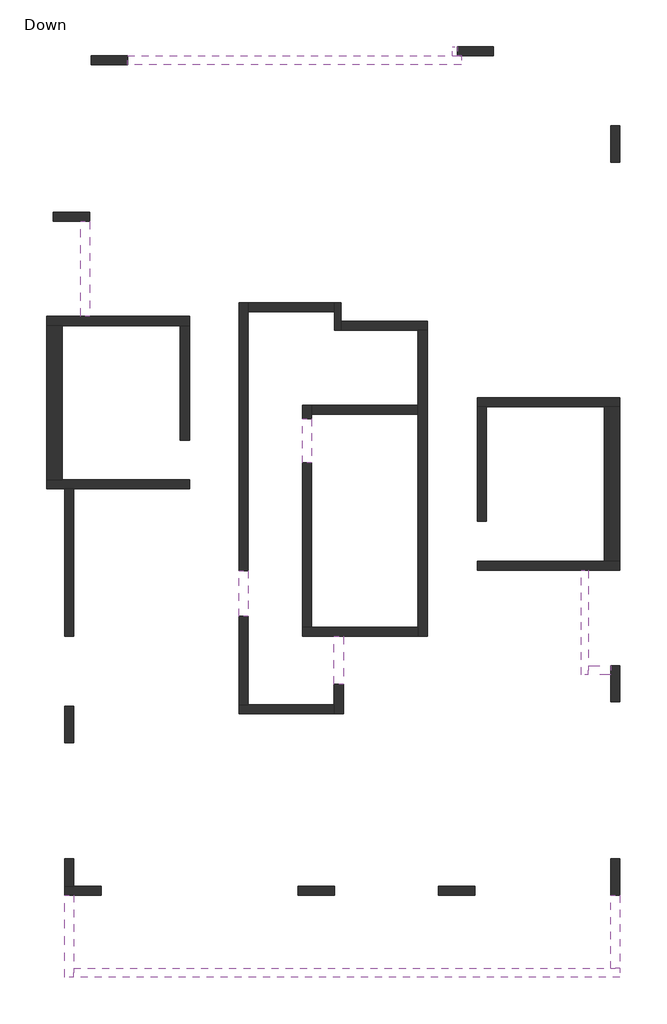
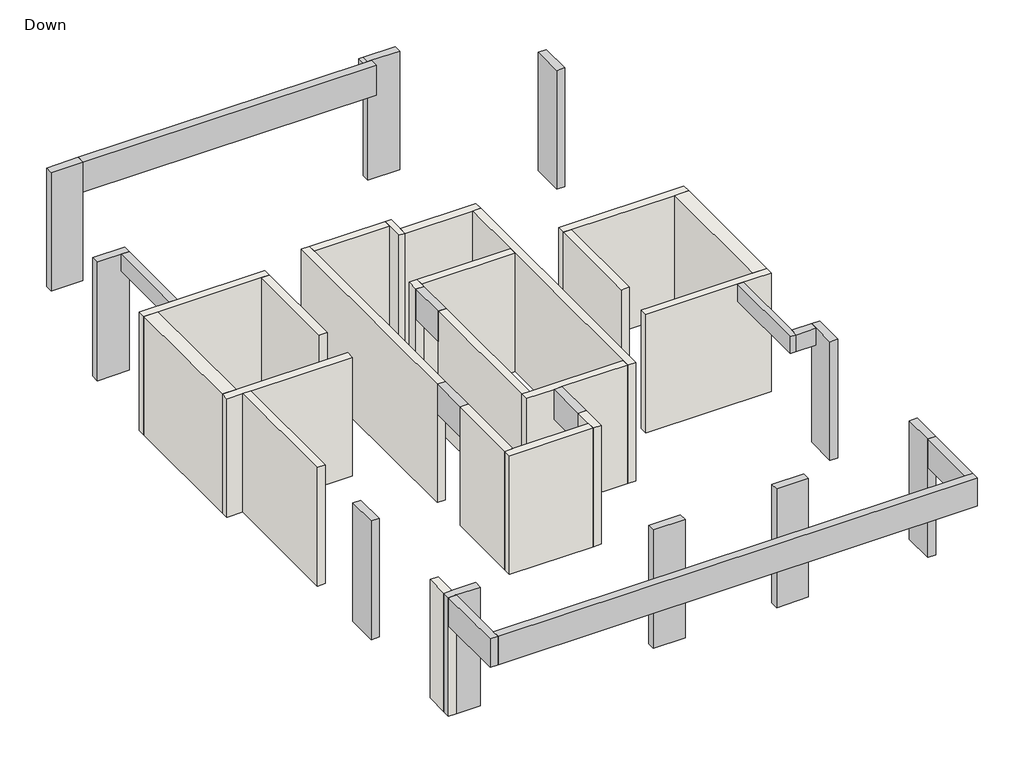
# One storey: 22 walls, 11 beams, 10 columns.
# Revit data of these elements (continued)
# Element 28 (IfcWall, "20") (continued)
#   SOFiSTiK_AMG_Adjusted = yes
#   Phase Created = New Construction
#   Base Constraint = Down
#   Top Constraint = Typical Floor
#   Materials on its faces: "Concrete"
# Element 29 (IfcWall, "20")
#   Comments = ""
#   Mark = "W8"
#   SOFiSTiK_EdgeZones = "W8"
#   SOFiSTiK_AMG_Comments = ""
#   Top Offset = 0 cm
#   Base Offset = 0 cm
#   wall height = 315 cm
#   SOFiSTiK_AMG_Scheduled = yes
#   SOFiSTiK_AMG_Adjusted = yes
#   Phase Created = New Construction
#   Base Constraint = Down
#   Top Constraint = Typical Floor
#   Materials on its faces: "Concrete"
# Element 30 (IfcWall, "20")
#   Comments = ""
#   Mark = "W9"
#   SOFiSTiK_EdgeZones = "W9"
#   SOFiSTiK_AMG_Comments = ""
#   Top Offset = 0 cm
#   Base Offset = 0 cm
#   wall height = 315 cm
#   SOFiSTiK_AMG_Scheduled = yes
#   SOFiSTiK_AMG_Adjusted = yes
#   Phase Created = New Construction
#   Base Constraint = Down
#   Top Constraint = Typical Floor
#   Materials on its faces: "Concrete"
# Element 31 (IfcWall, "20")
#   Comments = ""
#   Mark = "W10"
#   SOFiSTiK_EdgeZones = "W10"
#   SOFiSTiK_AMG_Comments = ""
#   Top Offset = 0 cm
#   Base Offset = 0 cm
#   wall height = 315 cm
#   SOFiSTiK_AMG_Scheduled = yes
#   SOFiSTiK_AMG_Adjusted = yes
#   Phase Created = New Construction
#   Base Constraint = Down
#   Top Constraint = Typical Floor
#   Materials on its faces: "Concrete"
# Element 32 (IfcWall, "20")
#   Comments = ""
#   Mark = "W11"
#   SOFiSTiK_EdgeZones = "W11"
#   SOFiSTiK_AMG_Comments = ""
#   Top Offset = 0 cm
#   Base Offset = 0 cm
#   wall height = 315 cm
#   SOFiSTiK_AMG_Scheduled = yes
#   SOFiSTiK_AMG_Adjusted = yes
#   Phase Created = New Construction
#   Base Constraint = Down
#   Top Constraint = Typical Floor
#   Materials on its faces: "Concrete"
# Element 33 (IfcWall, "20")
#   Comments = ""
#   Mark = "W12"
#   SOFiSTiK_EdgeZones = "W12"
#   SOFiSTiK_AMG_Comments = ""
#   Top Offset = 0 cm
#   Base Offset = 0 cm
#   wall height = 315 cm
#   SOFiSTiK_AMG_Scheduled = yes
#   SOFiSTiK_AMG_Adjusted = yes
#   Phase Created = New Construction
#   Base Constraint = Down
#   Top Constraint = Typical Floor
#   Materials on its faces: "Concrete"
# Element 34 (IfcWall, "20")
#   Comments = ""
#   Mark = "W13"
#   SOFiSTiK_EdgeZones = "W13"
#   SOFiSTiK_AMG_Comments = ""
#   Top Offset = 0 cm
#   Base Offset = 0 cm
#   wall height = 315 cm
#   SOFiSTiK_AMG_Scheduled = yes
#   SOFiSTiK_AMG_Adjusted = yes
#   Phase Created = New Construction
#   Base Constraint = Down
#   Top Constraint = Typical Floor
#   Materials on its faces: "Concrete"
# Element 35 (IfcWall, "20")
#   Comments = ""
#   Mark = "W14"
#   SOFiSTiK_EdgeZones = "W14"
#   SOFiSTiK_AMG_Comments = ""
#   Top Offset = 0 cm
#   Base Offset = 0 cm
#   wall height = 315 cm
#   SOFiSTiK_AMG_Scheduled = yes
#   SOFiSTiK_AMG_Adjusted = yes
#   Phase Created = New Construction
#   Base Constraint = Down
#   Top Constraint = Typical Floor
#   Materials on its faces: "Concrete"
# Element 36 (IfcWall, "20")
#   Comments = ""
#   Mark = "W15"
#   SOFiSTiK_EdgeZones = "W15"
#   SOFiSTiK_AMG_Comments = ""
#   Top Offset = 0 cm
#   Base Offset = 0 cm
#   wall height = 315 cm
#   SOFiSTiK_AMG_Scheduled = yes
#   SOFiSTiK_AMG_Adjusted = yes
#   Phase Created = New Construction
#   Base Constraint = Down
#   Top Constraint = Typical Floor
#   Materials on its faces: "Concrete"
# Element 37 (IfcWall, "20")
#   Comments = ""
#   Mark = "W16"
#   SOFiSTiK_EdgeZones = "W16"
#   SOFiSTiK_AMG_Comments = ""
#   Top Offset = 0 cm
#   Base Offset = 0 cm
#   wall height = 315 cm
#   SOFiSTiK_AMG_Scheduled = yes
#   SOFiSTiK_AMG_Adjusted = yes
#   Phase Created = New Construction
#   Base Constraint = Down
#   Top Constraint = Typical Floor
#   Materials on its faces: "Concrete"
# Element 38 (IfcWall, "20")
#   Comments = ""
#   Mark = "W17"
#   SOFiSTiK_EdgeZones = "W17"
#   SOFiSTiK_AMG_Comments = ""
#   Top Offset = 0 cm
#   Base Offset = 0 cm
#   wall height = 315 cm
#   SOFiSTiK_AMG_Scheduled = yes
#   SOFiSTiK_AMG_Adjusted = yes
#   Phase Created = New Construction
#   Base Constraint = Down
#   Top Constraint = Typical Floor
#   Materials on its faces: "Concrete"
# Element 39 (IfcWall, "20")
#   Comments = ""
#   Mark = "W18"
#   SOFiSTiK_EdgeZones = "W18"
#   SOFiSTiK_AMG_Comments = ""
#   Top Offset = 0 cm
#   Base Offset = 0 cm
#   wall height = 315 cm
#   SOFiSTiK_AMG_Scheduled = yes
#   SOFiSTiK_AMG_Adjusted = yes
#   Phase Created = New Construction
#   Base Constraint = Down
#   Top Constraint = Typical Floor
#   Materials on its faces: "Concrete"
# Element 40 (IfcWall, "20")
#   Comments = ""
#   Mark = "W19"
#   SOFiSTiK_EdgeZones = "W19"
#   SOFiSTiK_AMG_Comments = ""
#   Top Offset = 0 cm
#   Base Offset = 0 cm
#   wall height = 315 cm
#   SOFiSTiK_AMG_Scheduled = yes
#   SOFiSTiK_AMG_Adjusted = yes
#   Phase Created = New Construction
#   Base Constraint = Down
#   Top Constraint = Typical Floor
#   Materials on its faces: "Concrete"
# Element 41 (IfcWall, "20")
#   Comments = ""
#   Mark = "W21"
#   SOFiSTiK_EdgeZones = "W21"
#   SOFiSTiK_AMG_Comments = ""
#   Top Offset = 0 cm
#   Base Offset = 0 cm
#   wall height = 315 cm
#   SOFiSTiK_AMG_Scheduled = yes
#   SOFiSTiK_AMG_Adjusted = yes
#   Phase Created = New Construction
#   Base Constraint = Down
#   Top Constraint = Typical Floor
#   Materials on its faces: "Concrete"
# Element 42 (IfcWall, "35")
#   Comments = ""
#   Mark = "W22"
#   SOFiSTiK_EdgeZones = "W22"
#   SOFiSTiK_AMG_Comments = ""
#   Top Offset = 0 cm
#   Base Offset = 0 cm
#   wall height = 315 cm
#   SOFiSTiK_AMG_Scheduled = yes
#   SOFiSTiK_AMG_Adjusted = yes
#   Phase Created = New Construction
#   Base Constraint = Down
#   Top Constraint = Typical Floor
#   Materials on its faces: "Concrete"
# Element 43 (IfcWall, "35")
#   Comments = ""
#   Mark = "W23"
#   SOFiSTiK_EdgeZones = "W23"
#   SOFiSTiK_AMG_Comments = ""
#   Top Offset = 0 cm
#   Base Offset = 0 cm
#   wall height = 315 cm
#   SOFiSTiK_AMG_Scheduled = yes
#   SOFiSTiK_AMG_Adjusted = yes
#   Phase Created = New Construction
#   Base Constraint = Down
#   Top Constraint = Typical Floor
#   Materials on its faces: "Concrete"
# Materials
#   "Concrete": class "Concrete", colour RGB 192 192 192, transparency 0, Keynote = "01000", Description = "Cast-in-place concrete", Cost = 0
